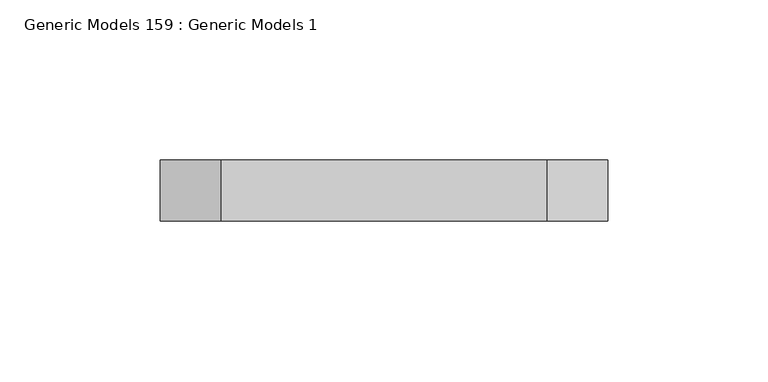
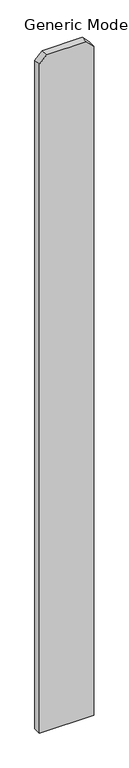
"""IFC4 building model written with IfcOpenShell, lengths in millimetres: proxy geometry, Generic Models 159 : Generic Models 1."""

from ifc_helpers import new_model, si_unit, frame, origin, place, context, project, spatial, polyline, outline, extrude, source, transform, mapped, element, save


def generic_models_159_generic_models_1_f226e3f2(model_context):
    return source(origin(), model_context, "Body", "SweptSolid", [
        extrude(outline(polyline([(76.2, -250572.5875), (1885.95, -250572.5875), (1905.0, -250591.6375), (1905.0, -250693.2375), (1885.95, -250712.2875), (76.2, -250712.2875), (76.2, -250572.5875)])), frame((0.0, 547.6875, 0.0), z_axis=(0.0, 1.0, 0.0), x_axis=(0.0, 0.0, 1.0)), (0.0, 0.0, 1.0), 19.05),
    ])


if __name__ == "__main__":
    model = new_model("IFC4")
    model_context = context("Model", 3, world=origin())
    ifc_project = project(units=[si_unit("LENGTHUNIT", "METRE", prefix="MILLI")], contexts=[model_context])
    site = spatial("IfcSite", under=ifc_project)
    building = spatial("IfcBuilding", under=site)
    placement = place(None, origin())
    generic_models_159_generic_models_1_shape = generic_models_159_generic_models_1_f226e3f2(model_context)
    element("IfcBuildingElementProxy", 1, Name="Generic Models 159 : Generic Models 1", ObjectType="Generic Models 159 : Generic Models 1", at=placement, inside=building, context=model_context, shape_type="MappedRepresentation", body=[
        mapped(generic_models_159_generic_models_1_shape, transform((0.0, 0.0, 0.0), x_axis=(1.0, 0.0, 0.0), y_axis=(0.0, 1.0, 0.0), z_axis=(0.0, 0.0, 1.0))),
    ])
    save(model, "model.ifc")

# Revit data of these elements
# Element 1 (IfcBuildingElementProxy, "Generic Models 159 : Generic Models 1")
#   Materials on its faces: "VERTICAL 1X6 CEDAR PLANKS W/ CLEAR WOOD SEALER"
# Materials
#   "VERTICAL 1X6 CEDAR PLANKS W/ CLEAR WOOD SEALER": class "Wood", colour RGB 234 198 147, transparency 0, Description = "Pinus Echinata", Cost = 0
